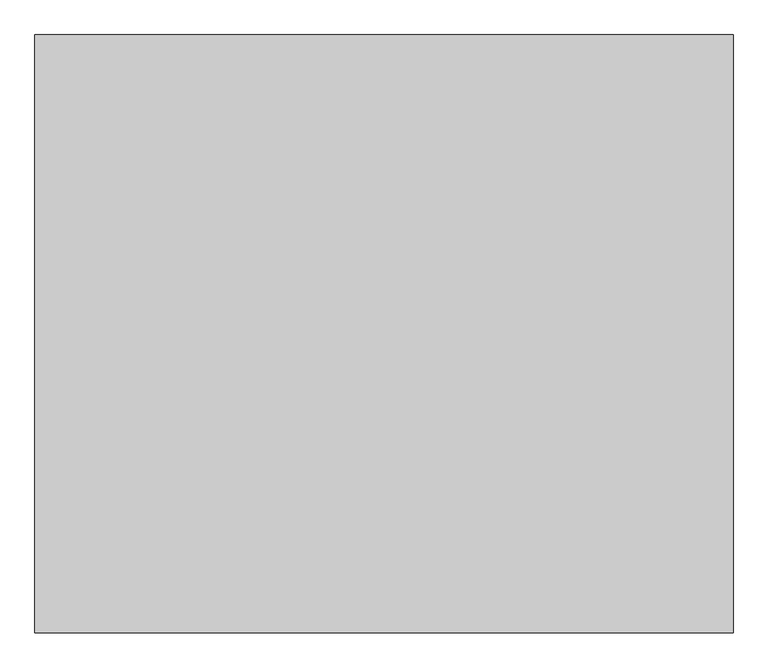
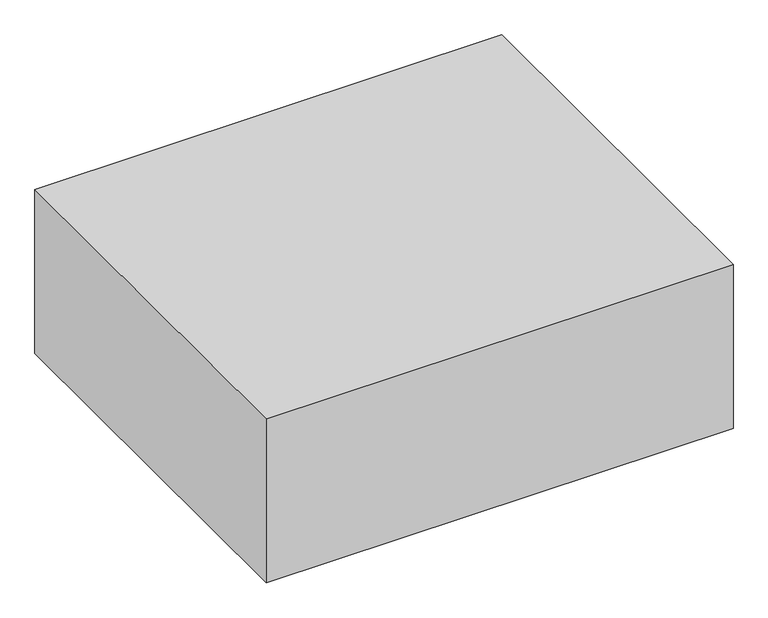
"""IFC4 building model written with IfcOpenShell, lengths in millimetres: proxy geometry, Space Planning Box_hec : Space Planning Box_hec."""

from ifc_helpers import new_model, si_unit, origin, origin_with_axes, place, context, project, spatial, polyline, outline, extrude, source, transform, mapped, element, save


def generic_models_ec4f78ea(model_context):
    return source(origin(), model_context, "Body", "SweptSolid", [
        extrude(outline(polyline([(7000.0, 6000.0), (7000.0, -6000.0), (-7000.0, -6000.0), (-7000.0, 6000.0), (7000.0, 6000.0)])), origin_with_axes(), (0.0, 0.0, 1.0), 5200.0),
    ])


if __name__ == "__main__":
    model = new_model("IFC4")
    model_context = context("Model", 3, world=origin())
    ifc_project = project(units=[si_unit("LENGTHUNIT", "METRE", prefix="MILLI")], contexts=[model_context])
    site = spatial("IfcSite", under=ifc_project)
    building = spatial("IfcBuilding", under=site)
    placement = place(None, origin())
    generic_models_shape = generic_models_ec4f78ea(model_context)
    element("IfcBuildingElementProxy", 1, Name="Space Planning Box_hec : Space Planning Box_hec", ObjectType="Space Planning Box_hec : Space Planning Box_hec", at=placement, inside=building, context=model_context, shape_type="MappedRepresentation", body=[
        mapped(generic_models_shape, transform((0.0, 0.0, 0.0), x_axis=(1.0, 0.0, 0.0), y_axis=(0.0, 1.0, 0.0), z_axis=(0.0, 0.0, 1.0))),
    ])
    save(model, "model.ifc")

# Revit data of these elements
# Type "Space Planning Box_hec : Space Planning Box_hec"
#   Type Comments = "..."
#   Room Name [instance default] = "?"
#   Interior Finish [instance default] = ""
#   Exterior Finish [instance default] = ""
#   Department [instance default] = ""
#   Assembly Code = "..."
#   ceiling height [instance default] = 0
#   Width [instance default] = 1524 mm
#   Program Area [instance default] = 0.00 m²
#   Length [instance default] = 1524 mm
#   Height [instance default] = 1524 mm
#   Area [instance default] = 2.32258 m²
#   Fill Color [instance default] = Cyan
#   Default Elevation = 0
# Element 1 (IfcBuildingElementProxy, "Space Planning Box_hec : Space Planning Box_hec")
#   Room Name = "Battery Room"
#   Interior Finish = "IW2..N/A,,WB4..N/A,,FL3..N/A,,CL2..N/A"
#   Exterior Finish = "N/A..N/A,,EW1..N/A"
#   Department = "EL"
#   Width = 14000 mm
#   Program Area = 168.00 m²
#   Length = 12000 mm
#   Height = 5200 mm
#   Area = 168.00 m²
#   Fill Color = Orange
#   Materials on its faces: "Orange"
# Materials
#   "Cyan": class "Generic", colour RGB 0 255 255, transparency 0.2, Cost = 0
#   "Orange": class "Generic", colour RGB 255 165 0, transparency 0.2, Cost = 0
